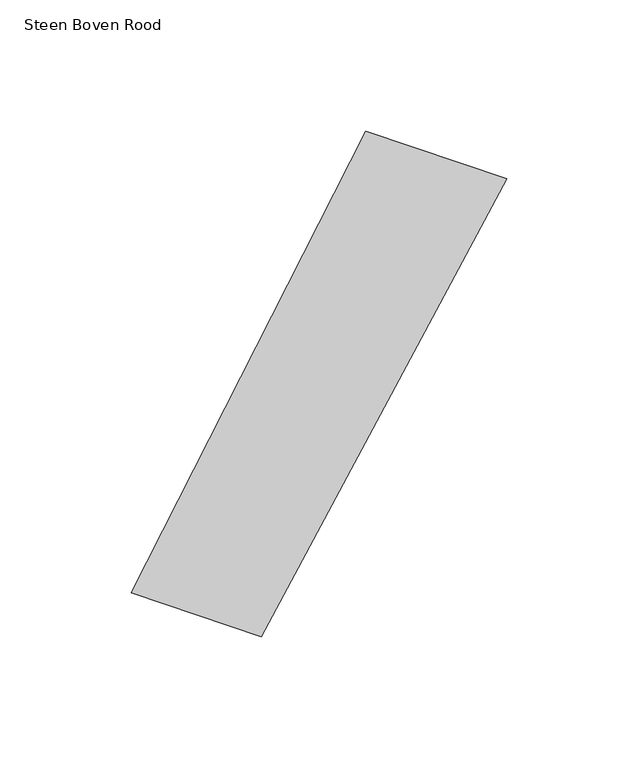
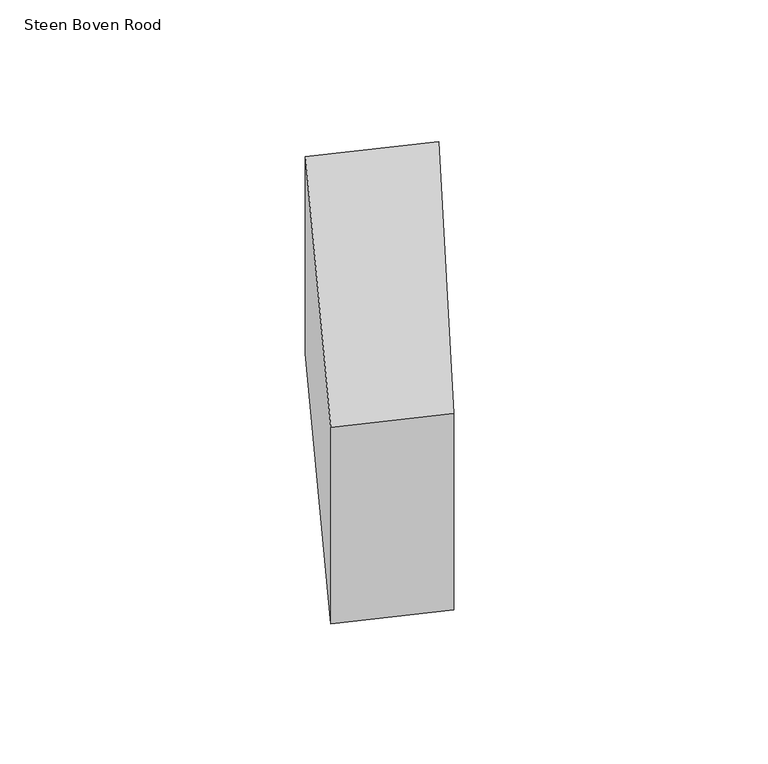
"""IFC4 building model written with IfcOpenShell, lengths in millimetres: proxy geometry, 00_GMA_steen_versie_4 : Steen Boven Rood."""

from ifc_helpers import new_model, si_unit, origin, origin_with_axes, place, context, project, spatial, polyline, outline, extrude, source, transform, mapped, element, save


def steen_boven_rood_31ec0a7c(model_context):
    return source(origin(), model_context, "Body", "SweptSolid", [
        extrude(outline(polyline([(148.6837421, 159.5680602), (55.3122513, -14.7585486), (5.7532008, 2.0422921), (95.0121939, 177.7470595), (148.6837421, 159.5680602)])), origin_with_axes(), (0.0, 0.0, 1.0), 100.0),
    ])


if __name__ == "__main__":
    model = new_model("IFC4")
    model_context = context("Model", 3, world=origin())
    ifc_project = project(units=[si_unit("LENGTHUNIT", "METRE", prefix="MILLI")], contexts=[model_context])
    site = spatial("IfcSite", under=ifc_project)
    building = spatial("IfcBuilding", under=site)
    placement = place(None, origin())
    steen_boven_rood_shape = steen_boven_rood_31ec0a7c(model_context)
    element("IfcBuildingElementProxy", 1, Name="00_GMA_steen_versie_4 : Steen Boven Rood", ObjectType="00_GMA_steen_versie_4 : Steen Boven Rood", at=placement, inside=building, context=model_context, shape_type="MappedRepresentation", body=[
        mapped(steen_boven_rood_shape, transform((0.0, 0.0, 0.0), x_axis=(1.0, 0.0, 0.0), y_axis=(0.0, 1.0, 0.0), z_axis=(0.0, 0.0, 1.0))),
    ])
    save(model, "model.ifc")

# Revit data of these elements
# Type "00_GMA_steen_versie_4 : Steen Boven Rood"
#   StootVoegHalfBoven [instance default] = 5 mm
#   StootVoegHalf [instance default] = 5 mm
#   StootVoegBreedteOnder = 10 mm
#   StootVoegBreedteBoven = 10 mm
#   Steendikte = 100 mm
#   LintVoegOnderHalf = 5 mm
#   LintVoegOnder = 10 mm
#   LintVoegBovenHalf = 0 mm
#   LintVoegBoven = 0 mm
#   materiaal = 21_steen_rood
#   MateriaalVoeg = none
#   Default Elevation = 0
# Element 1 (IfcBuildingElementProxy, "00_GMA_steen_versie_4 : Steen Boven Rood")
#   Materials on its faces: "21_steen_rood"
# Materials
#   "21_steen_rood": class "Unassigned", colour RGB 213 111 43, transparency 0, Cost = 0
